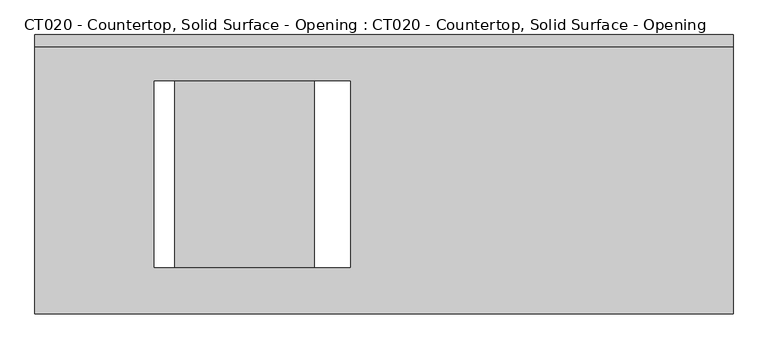
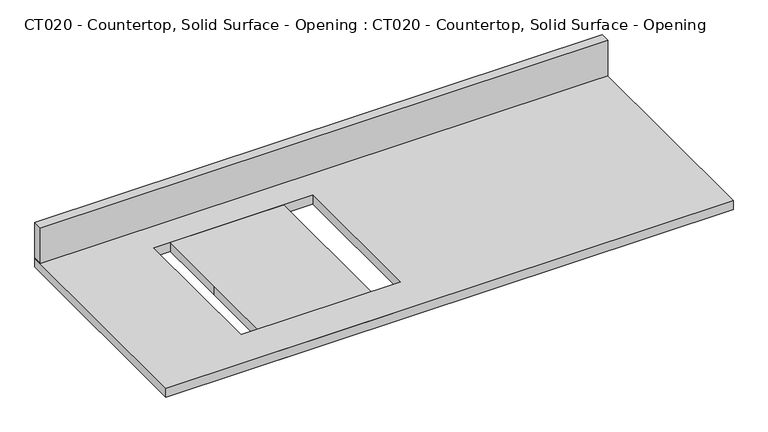
"""IFC4 building model written with IfcOpenShell, lengths in millimetres: proxy geometry, CT020 - Countertop, Solid Surface - Opening : CT020 - Countertop, Solid Surface - Opening."""

import ifcopenshell
import ifcopenshell.guid

model = None  # the IFC model being written
_history = None  # IfcOwnerHistory: only IFC2X3 demands one
_inside = {}  # id of a spatial element -> (the spatial element, [elements in it])
_under = {}  # id of a project, library or spatial element -> (it, [spatial elements below it])
_declared = {}  # id of a project -> (the project, [libraries it declares])
_typed = {}  # id of a type object -> (the type object, [elements of that type])
_made_of = {}  # id of a material, layer set ... -> (it, [elements and type objects made of it])


def new_model(schema):
    """Start an empty IFC model of exactly this schema.

    Asked for "IFC4X3", IfcOpenShell would pick the latest addendum, in which some entities
    have other attributes; the version numbers below select the first issue.
    IFC2X3 requires an IfcOwnerHistory on every rooted entity: one is made here for all.
    """
    global model, _history
    if schema == "IFC4X3":
        model = ifcopenshell.file(schema_version=(4, 3, 0, 0))
    else:
        model = ifcopenshell.file(schema=schema)
    _inside.clear()
    _under.clear()
    _declared.clear()
    _typed.clear()
    _made_of.clear()
    _history = None
    if model.schema == "IFC2X3":
        org = make("IfcOrganization", Name="unknown")
        user = make(
            "IfcPersonAndOrganization",
            ThePerson=make("IfcPerson", FamilyName="unknown"),
            TheOrganization=org,
        )
        app = make(
            "IfcApplication",
            ApplicationDeveloper=org,
            Version="unknown",
            ApplicationFullName="unknown",
            ApplicationIdentifier="unknown",
        )
        _history = make(
            "IfcOwnerHistory",
            OwningUser=user,
            OwningApplication=app,
            ChangeAction="ADDED",
            CreationDate=0,
        )
    return model


def make(cls, **values):
    """One entity of the class cls with the attributes given. An attribute that is None is left unset."""
    return model.create_entity(
        cls, **{name: value for name, value in values.items() if value is not None}
    )


def rooted(cls, **values):
    """An entity with a GlobalId (a new one), such as an element, a storey or a relation."""
    return make(cls, GlobalId=ifcopenshell.guid.new(), OwnerHistory=_history, **values)


def si_unit(unit_type, name, prefix=None):
    """IfcSIUnit, for example si_unit("LENGTHUNIT", "METRE", prefix="MILLI")."""
    return make("IfcSIUnit", UnitType=unit_type, Prefix=prefix, Name=name)


def assignment(units):
    """IfcUnitAssignment: the units of a project."""
    return None if units is None else make("IfcUnitAssignment", Units=units)


def point(xyz):
    """IfcCartesianPoint."""
    return None if xyz is None else make("IfcCartesianPoint", Coordinates=xyz)


def direction(xyz):
    """IfcDirection."""
    return None if xyz is None else make("IfcDirection", DirectionRatios=xyz)


def frame(location, z_axis=None, x_axis=None):
    """IfcAxis2Placement3D, a coordinate frame: its origin and axes. An axis left out is left unset."""
    return make(
        "IfcAxis2Placement3D",
        Location=point(location),
        Axis=direction(z_axis),
        RefDirection=direction(x_axis),
    )


def origin():
    """The frame at (0, 0, 0) with its axes left unset."""
    return frame((0.0, 0.0, 0.0))


def origin_with_axes():
    """The frame at (0, 0, 0) with the z axis (0, 0, 1) and the x axis (1, 0, 0) written out."""
    return frame((0.0, 0.0, 0.0), z_axis=(0.0, 0.0, 1.0), x_axis=(1.0, 0.0, 0.0))


def place(relative_to, where):
    """IfcLocalPlacement: puts the frame where relative to a parent placement (None: the world)."""
    return make(
        "IfcLocalPlacement", PlacementRelTo=relative_to, RelativePlacement=where
    )


def context(
    kind, dimensions, precision=None, world=None, true_north=None, identifier=None
):
    """IfcGeometricRepresentationContext, for example the 3D "Model" context."""
    return make(
        "IfcGeometricRepresentationContext",
        ContextIdentifier=identifier,
        ContextType=kind,
        CoordinateSpaceDimension=dimensions,
        Precision=precision,
        WorldCoordinateSystem=world,
        TrueNorth=true_north,
    )


def project(units=None, contexts=None):
    """IfcProject with its units and contexts."""
    return rooted(
        "IfcProject",
        Name="project",
        RepresentationContexts=contexts,
        UnitsInContext=assignment(units),
    )


def spatial(cls, under=None, at=None, **own):
    """A site, building, storey or space (cls), placed at a placement, below another one or the project."""
    s = rooted(cls, ObjectPlacement=at, **own)
    if under is not None:
        _under.setdefault(under.id(), (under, []))[1].append(s)
    return s


def polyline(points):
    """IfcPolyline through the points."""
    return make("IfcPolyline", Points=[point(p) for p in points])


def outline(outer, holes=None, kind="AREA"):
    """IfcArbitraryClosedProfileDef: a profile drawn as a closed curve; with holes, ...WithVoids."""
    if holes is None:
        return make("IfcArbitraryClosedProfileDef", ProfileType=kind, OuterCurve=outer)
    return make(
        "IfcArbitraryProfileDefWithVoids",
        ProfileType=kind,
        OuterCurve=outer,
        InnerCurves=holes,
    )


def extrude(swept, where, along, depth):
    """IfcExtrudedAreaSolid: the profile swept, set in the frame where, extruded along a direction by depth."""
    return make(
        "IfcExtrudedAreaSolid",
        SweptArea=swept,
        Position=where,
        ExtrudedDirection=direction(along),
        Depth=depth,
    )


def shape(context_of_items, identifier, shape_type, items):
    """IfcShapeRepresentation: the items that make up one representation, for example the "Body"."""
    return make(
        "IfcShapeRepresentation",
        ContextOfItems=context_of_items,
        RepresentationIdentifier=identifier,
        RepresentationType=shape_type,
        Items=items,
    )


def source(mapping_origin, context_of_items, identifier, shape_type, items):
    """IfcRepresentationMap: a shape defined once, which mapped items show again and again."""
    return make(
        "IfcRepresentationMap",
        MappingOrigin=mapping_origin,
        MappedRepresentation=shape(context_of_items, identifier, shape_type, items),
    )


def transform(
    local_origin,
    x_axis=None,
    y_axis=None,
    z_axis=None,
    scale=None,
    scale2=None,
    scale3=None,
    uniform=True,
):
    """IfcCartesianTransformationOperator3D, or its non-uniform kind. x_axis, y_axis, z_axis: its Axis1, 2, 3."""
    if uniform:
        return make(
            "IfcCartesianTransformationOperator3D",
            Axis1=direction(x_axis),
            Axis2=direction(y_axis),
            LocalOrigin=point(local_origin),
            Scale=scale,
            Axis3=direction(z_axis),
        )
    return make(
        "IfcCartesianTransformationOperator3DnonUniform",
        Axis1=direction(x_axis),
        Axis2=direction(y_axis),
        LocalOrigin=point(local_origin),
        Scale=scale,
        Axis3=direction(z_axis),
        Scale2=scale2,
        Scale3=scale3,
    )


def mapped(mapping_source, mapping_target):
    """IfcMappedItem: shows the shape of a source again, moved by a transform."""
    return make(
        "IfcMappedItem", MappingSource=mapping_source, MappingTarget=mapping_target
    )


def made_of(thing, what):
    """Note that an element or type object is made of a material, layer set ...; save() writes the relation."""
    if what is not None:
        _made_of.setdefault(what.id(), (what, []))[1].append(thing)
    return thing


def element(
    cls,
    number,
    at=None,
    inside=None,
    cuts=None,
    type_object=None,
    material=None,
    context=None,
    identifier="Body",
    shape_type=None,
    held_by="IfcProductDefinitionShape",
    body=None,
    shapes=None,
    **own,
):
    """One element of the class cls, such as IfcWall. Its Tag is "e" and its number.

    at: its placement. inside: the storey or other place that contains it. cuts: it is an
    opening in that element (IfcRelVoidsElement). A single representation is given by context,
    identifier, shape_type and body (its items); several are given by shapes. held_by: the class
    of the entity that holds the representations. save() writes the other relations.
    """
    e = rooted(cls, Tag="e%d" % number, ObjectPlacement=at, **own)
    if body is not None:
        shapes = [shape(context, identifier, shape_type, body)]
    if shapes is not None:
        e.Representation = make(held_by, Representations=shapes)
    if inside is not None:
        _inside.setdefault(inside.id(), (inside, []))[1].append(e)
    if cuts is not None:
        rooted(
            "IfcRelVoidsElement", RelatingBuildingElement=cuts, RelatedOpeningElement=e
        )
    if type_object is not None:
        _typed.setdefault(type_object.id(), (type_object, []))[1].append(e)
    return made_of(e, material)


def aggregate(whole, parts):
    """IfcRelAggregates: a whole, such as a stair, and the parts it consists of."""
    return rooted("IfcRelAggregates", RelatingObject=whole, RelatedObjects=parts)


def save(model, path):
    """Write the relations noted so far, then the file.

    IfcRelAggregates (storeys below a building ...), IfcRelContainedInSpatialStructure (elements
    in a storey), IfcRelDefinesByType, IfcRelAssociatesMaterial and IfcRelDeclares: one each for
    every whole, place, type object, material and project.
    """
    for whole, parts in _under.values():
        aggregate(whole, parts)
    for where, things in _inside.values():
        rooted(
            "IfcRelContainedInSpatialStructure",
            RelatedElements=things,
            RelatingStructure=where,
        )
    for kind, things in _typed.values():
        rooted("IfcRelDefinesByType", RelatedObjects=things, RelatingType=kind)
    for what, things in _made_of.values():
        rooted("IfcRelAssociatesMaterial", RelatedObjects=things, RelatingMaterial=what)
    for by, libraries in _declared.values():
        rooted("IfcRelDeclares", RelatingContext=by, RelatedDefinitions=libraries)
    model.write(path)


def ct020_countertop_solid_surface_opening_ct020_countertop_3d6740ce(model_context):
    return source(origin(), model_context, "Body", "SweptSolid", [
        extrude(outline(polyline([(1066.8, 304.8), (1066.8, -304.8), (-457.2, -304.8), (-457.2, 304.8), (1066.8, 304.8)]), holes=[polyline([(230.9825513, 203.2), (-196.5490426, 203.2), (-196.5490426, -203.2), (230.9825513, -203.2), (230.9825513, 203.2)])]), origin_with_axes(), (0.0, 0.0, 1.0), 25.4),
        extrude(outline(polyline([(-457.2, 279.4), (-457.2, 304.8), (1066.8, 304.8), (1066.8, 279.4), (-457.2, 279.4)])), frame((0.0, 0.0, 25.4), z_axis=(0.0, 0.0, 1.0), x_axis=(1.0, 0.0, 0.0)), (0.0, 0.0, 1.0), 101.6),
        extrude(outline(polyline([(-152.4, 304.8), (152.4, 304.8), (152.4, -304.8), (-152.4, -304.8), (-152.4, 0.0), (-152.4, 304.8)])), origin_with_axes(), (0.0, 0.0, 1.0), 25.4),
    ])


if __name__ == "__main__":
    model = new_model("IFC4")
    model_context = context("Model", 3, world=origin())
    ifc_project = project(units=[si_unit("LENGTHUNIT", "METRE", prefix="MILLI")], contexts=[model_context])
    site = spatial("IfcSite", under=ifc_project)
    building = spatial("IfcBuilding", under=site)
    placement = place(None, origin())
    ct020_countertop_solid_surface_opening_ct020_countertop_shape = ct020_countertop_solid_surface_opening_ct020_countertop_3d6740ce(model_context)
    element("IfcBuildingElementProxy", 1, Name="CT020 - Countertop, Solid Surface - Opening : CT020 - Countertop, Solid Surface - Opening", ObjectType="CT020 - Countertop, Solid Surface - Opening : CT020 - Countertop, Solid Surface - Opening", at=placement, inside=building, context=model_context, shape_type="MappedRepresentation", body=[
        mapped(ct020_countertop_solid_surface_opening_ct020_countertop_shape, transform((0.0, 0.0, 0.0), x_axis=(1.0, 0.0, 0.0), y_axis=(0.0, 1.0, 0.0), z_axis=(0.0, 0.0, 1.0))),
    ])
    save(model, "model.ifc")

# Revit data of these elements
# Project information
#   Room Abbreviation = "OPIR1"
#   Room Description = "Immunizations (OPIR1)"
#   Sheets - Total = "5"
#   Project Issue Date = "Issue Date"
#   Project Status = "Project Status"
#   Client Name = "Owner"
#   Project Address = "Enter address here"
#   Project Name = "Project Name"
#   Project Number = "Project Number"
#   Publication Date = "1-Feb-16"
# Type "CT020 - Countertop, Solid Surface - Opening : CT020 - Countertop, Solid Surface - Opening"
#   JSN = "CT020"
#   Nomenclature = "Countertop, Solid Surface"
#   UTIL_1_WaterDrain = "-"
#   UTIL_2_Elec = "-"
#   UTIL_3_MedGas = "-"
#   UTIL_4_MiscGas = "-"
#   UTIL_5_NonMedGas = "-"
#   UTIL_6_Misc = "-"
#   Utility_6 = "-"
#   Utility_5 = "-"
#   Utility_4 = "-"
#   Utility_3 = "-"
#   Utility_2 = "-"
#   Utility_1 = "-"
#   Unit_Issue = "LF"
#   Price_Date = "12/05/2012"
#   Nomenclature = "Countertop, Solid Surface"
#   NSN = "6530"
#   Location [instance default] = ""
#   JSN_Name = "CT020"
#   Hertz_swit = "0"
#   Hertz_dep = "0"
#   Hertz = "0"
#   Desc = "A solid, nonporous countertop with a smooth seamless appearance. Easy to clean and maintain and with proper cleaning does not support the growth of mold. An acrylic-based solid surface product. Standard thickness of 1\", and a 4\" butt backsplash/curb. Also referred to as a work surface or work top. Available in a choice of colors and depths. Used in lab and other hospital areas requiring optimum physical and chemical resisting properties."
#   CAT_VA = "-"
#   CAT_Navy = "A"
#   CAT_IHS = "A"
#   CAT_Army = "A"
#   CAT_AF = "-"
#   BTUPerHour = "0"
#   Width_IN = 12
#   Weight_AV = 0
#   Watts2 = 0
#   Watts1 = 0
#   Volts2 = 0
#   Volts1 = 0
#   Phase2 = 0
#   Phase1 = 0
#   OpeningLength2 [instance default] = 1' - 6"
#   OpeningLength [instance default] = 2' - 0"
#   OpeningDepth2 [instance default] = 0' - 8"
#   OpeningDepth [instance default] = 0' - 8"
#   Height_IN = 5
#   Depth_IN = 30
#   CustomLength2 [instance default] = 3' - 0"
#   CustomLength [instance default] = 6' - 0"
#   Amps2 = 0
#   Amps1 = 0
#   Assembly Code = ""
# Element 1 (IfcBuildingElementProxy, "CT020 - Countertop, Solid Surface - Opening : CT020 - Countertop, Solid Surface - Opening")
#   OpeningLength2 = 0' - 9.0938"
#   OpeningLength = 0' - 7.73815"
#   CustomLength2 = 3' - 6"
#   CustomLength = 1' - 6"
#   Materials on its faces: "CounterTopFinish", "EquipSpace"
# Materials
#   "CounterTopFinish": class "Unassigned", colour RGB 139 121 96, transparency 0
#   "EquipSpace": class "Unassigned", colour RGB 221 217 195, transparency 0.5
